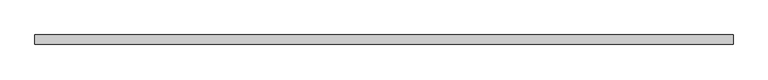
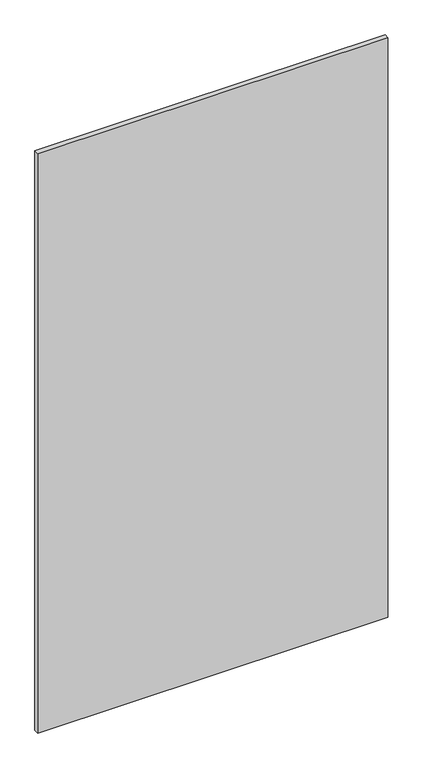
"""IFC4 building model written with IfcOpenShell, lengths in millimetres: plate geometry, 系统嵌板 : 玻璃."""

from ifc_helpers import new_model, si_unit, origin, origin_with_axes, place, context, project, spatial, polyline, outline, extrude, source, transform, mapped, element, save


def plate_751a20d5(model_context):
    return source(origin(), model_context, "Body", "SweptSolid", [
        extrude(outline(polyline([(915.0, -12.5), (-915.0, -12.5), (-915.0, 12.5), (915.0, 12.5), (915.0, -12.5)])), origin_with_axes(), (0.0, 0.0, 1.0), 3200.0),
    ])


if __name__ == "__main__":
    model = new_model("IFC4")
    model_context = context("Model", 3, world=origin())
    ifc_project = project(units=[si_unit("LENGTHUNIT", "METRE", prefix="MILLI")], contexts=[model_context])
    site = spatial("IfcSite", under=ifc_project)
    building = spatial("IfcBuilding", under=site)
    placement = place(None, origin())
    plate_shape = plate_751a20d5(model_context)
    element("IfcPlate", 1, ObjectType="系统嵌板 : 玻璃", at=placement, inside=building, context=model_context, shape_type="MappedRepresentation", body=[
        mapped(plate_shape, transform((0.0, 0.0, 0.0), x_axis=(1.0, 0.0, 0.0), y_axis=(0.0, 1.0, 0.0), z_axis=(0.0, 0.0, 1.0))),
    ])
    save(model, "model.ifc")

# Revit data of these elements
# Type "系统嵌板 : 玻璃"
#   Construction Type Id = "GSP4R"
#   Analytic Construction = "1/8 英寸 Pilkington 单层玻璃"
#   Visual Light Transmittance = 0.9
#   Solar Heat Gain Coefficient = 0.86
#   Heat Transfer Coefficient (U) = 6.7069 W/(m²·K)
# Element 1 (IfcPlate, "系统嵌板 : 玻璃")
#   Materials on its faces: "玻璃"
# Materials
#   "玻璃": class "玻璃", colour RGB 0 128 192, transparency 0.9, Description = "钠钙玻璃", Cost = 0
